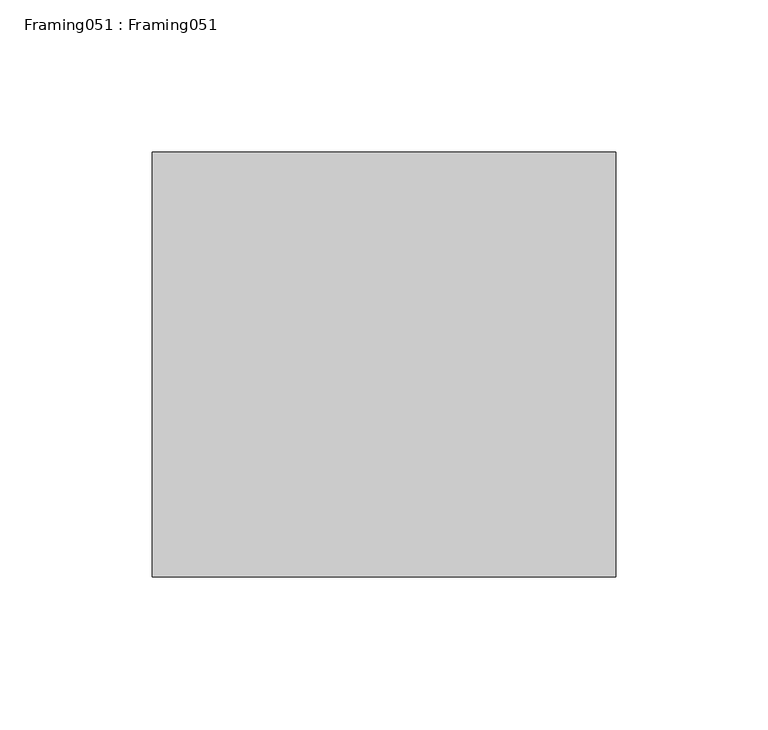
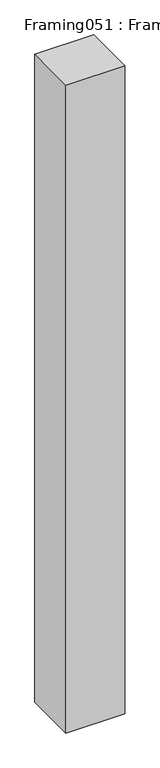
"""IFC4 building model written with IfcOpenShell, lengths in millimetres: proxy geometry, Framing051 : Framing051."""

from ifc_helpers import new_model, si_unit, frame, origin, place, context, project, spatial, polyline, outline, extrude, source, transform, mapped, element, save


def framing051_framing051_04a74bc1(model_context):
    return source(origin(), model_context, "Body", "SweptSolid", [
        extrude(outline(polyline([(12383.0178845, -4637.5417972), (12383.0178845, -4497.8425368), (12535.4178845, -4497.8425368), (12535.4178845, -4637.5417972), (12383.0178845, -4637.5417972)])), frame((0.0, 0.0, 36582.096), z_axis=(0.0, 0.0, 1.0), x_axis=(1.0, 0.0, 0.0)), (0.0, 0.0, 1.0), 1778.0),
    ])


if __name__ == "__main__":
    model = new_model("IFC4")
    model_context = context("Model", 3, world=origin())
    ifc_project = project(units=[si_unit("LENGTHUNIT", "METRE", prefix="MILLI")], contexts=[model_context])
    site = spatial("IfcSite", under=ifc_project)
    building = spatial("IfcBuilding", under=site)
    placement = place(None, origin())
    framing051_framing051_shape = framing051_framing051_04a74bc1(model_context)
    element("IfcBuildingElementProxy", 1, Name="Framing051 : Framing051", ObjectType="Framing051 : Framing051", at=placement, inside=building, context=model_context, shape_type="MappedRepresentation", body=[
        mapped(framing051_framing051_shape, transform((0.0, 0.0, 0.0), x_axis=(1.0, 0.0, 0.0), y_axis=(0.0, 1.0, 0.0), z_axis=(0.0, 0.0, 1.0))),
    ])
    save(model, "model.ifc")

# Revit data of these elements
# Type "Framing051 : Framing051"
#   NameOverride = "Framing051"
# Element 1 (IfcBuildingElementProxy, "Framing051 : Framing051")
#   Materials on its faces: "WOOD FRAMING (SEE STRUCT DWGS)"
# Materials
#   "WOOD FRAMING (SEE STRUCT DWGS)": class "Unassigned", colour RGB 224 188 168, transparency 0, Cost = 0
